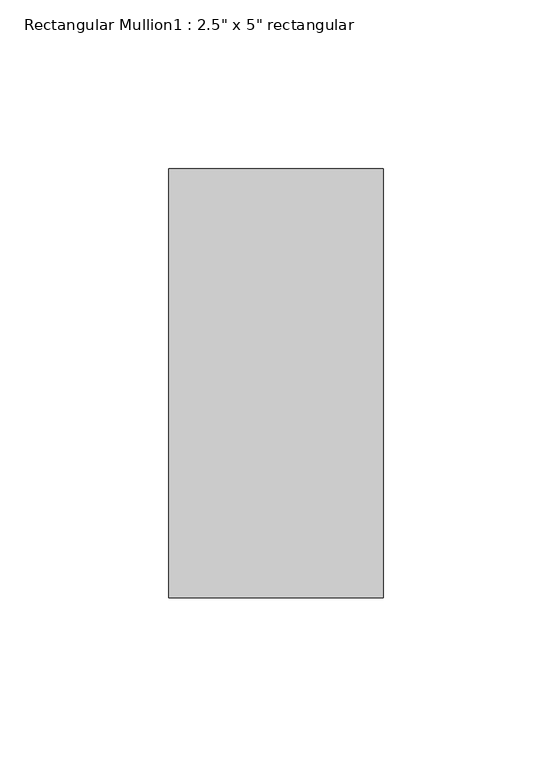
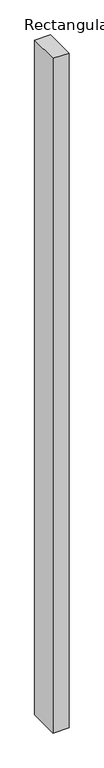
"""IFC4 building model written with IfcOpenShell, lengths in millimetres: member geometry."""

from ifc_helpers import new_model, si_unit, frame, origin, place, context, project, spatial, polyline, outline, extrude, source, transform, mapped, element, save


def member_5da9506a(model_context):
    return source(origin(), model_context, "Body", "SweptSolid", [
        extrude(outline(polyline([(0.0, 63.5), (0.0, -63.5), (-63.5, -63.5), (-63.5, 63.5), (0.0, 63.5)])), frame((0.0, 0.0, -2852.42), z_axis=(0.0, 0.0, 1.0), x_axis=(1.0, 0.0, 0.0)), (0.0, 0.0, 1.0), 2852.42),
    ])


if __name__ == "__main__":
    model = new_model("IFC4")
    model_context = context("Model", 3, world=origin())
    ifc_project = project(units=[si_unit("LENGTHUNIT", "METRE", prefix="MILLI")], contexts=[model_context])
    site = spatial("IfcSite", under=ifc_project)
    building = spatial("IfcBuilding", under=site)
    placement = place(None, origin())
    member_shape = member_5da9506a(model_context)
    element("IfcMember", 1, ObjectType="Rectangular Mullion1 : 2.5\" x 5\" rectangular", at=placement, inside=building, context=model_context, shape_type="MappedRepresentation", body=[
        mapped(member_shape, transform((0.0, 0.0, 0.0), x_axis=(1.0, 0.0, 0.0), y_axis=(0.0, 1.0, 0.0), z_axis=(0.0, 0.0, 1.0))),
    ])
    save(model, "model.ifc")

# Revit data of these elements
# Type "Rectangular Mullion1 : 2.5\" x 5\" rectangular"
#   built-in parameter 1007304 = 0.416667 (stored number, unit not read)
#   built-in parameter 1007301 = 0.104167 (stored number, unit not read)
#   built-in parameter 1007300 = 0.104167 (stored number, unit not read)
# Element 1 (IfcMember, "Rectangular Mullion1 : 2.5\" x 5\" rectangular")
#   Materials on its faces: "support-frame"
# Materials
#   "support-frame": class "Unassigned", colour RGB 233 233 233, transparency 0, Cost = 0
